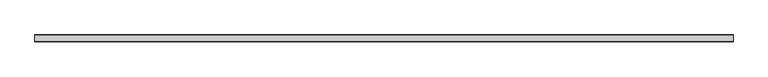
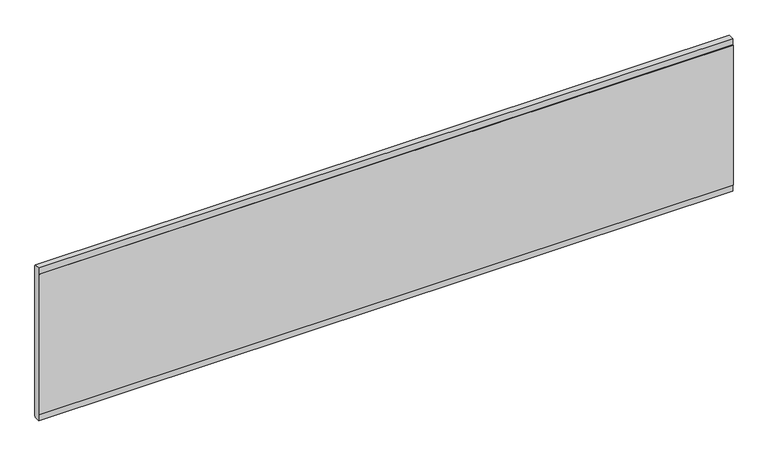
"""IFC4 building model written with IfcOpenShell, lengths in millimetres: proxy geometry, Stucco010 3062 : Stucco010 3062."""

from ifc_helpers import new_model, si_unit, frame, origin, place, context, project, spatial, polyline, outline, extrude, source, transform, mapped, element, save


def generic_models_abc11cbf(model_context):
    return source(origin(), model_context, "Body", "SweptSolid", [
        extrude(outline(polyline([(10464.4562552, 42924.8794763), (10464.4562552, 42921.3996763), (10447.4923073, 42921.3996763), (10447.4923073, 42940.4496763), (10446.2223073, 42940.4496763), (10446.2223073, 43367.3370312), (10447.4923073, 43367.3370312), (10447.4923073, 43386.3870313), (10464.4562552, 43386.3870313), (10464.4562552, 43382.9072312), (10465.7262552, 43382.9072312), (10465.7262552, 42924.8794763), (10464.4562552, 42924.8794763)])), frame((3694.2883192, 0.0, 0.0), z_axis=(1.0, 0.0, 0.0), x_axis=(0.0, 1.0, 0.0)), (0.0, 0.0, 1.0), 2000.0),
    ])


if __name__ == "__main__":
    model = new_model("IFC4")
    model_context = context("Model", 3, world=origin())
    ifc_project = project(units=[si_unit("LENGTHUNIT", "METRE", prefix="MILLI")], contexts=[model_context])
    site = spatial("IfcSite", under=ifc_project)
    building = spatial("IfcBuilding", under=site)
    placement = place(None, origin())
    generic_models_shape = generic_models_abc11cbf(model_context)
    element("IfcBuildingElementProxy", 1, Name="Stucco010 3062 : Stucco010 3062", ObjectType="Stucco010 3062 : Stucco010 3062", at=placement, inside=building, context=model_context, shape_type="MappedRepresentation", body=[
        mapped(generic_models_shape, transform((0.0, 0.0, 0.0), x_axis=(1.0, 0.0, 0.0), y_axis=(0.0, 1.0, 0.0), z_axis=(0.0, 0.0, 1.0))),
    ])
    save(model, "model.ifc")

# Revit data of these elements
# Type "Stucco010 3062 : Stucco010 3062"
#   NameOverride = "Stucco010"
# Element 1 (IfcBuildingElementProxy, "Stucco010 3062 : Stucco010 3062")
#   Materials on its faces: "7/8\" SMOOTH TROWEL EXTERIOR STUCCO"
# Materials
#   "7/8\" SMOOTH TROWEL EXTERIOR STUCCO": class "Unassigned", colour RGB 255 255 255, transparency 0, Cost = 0
